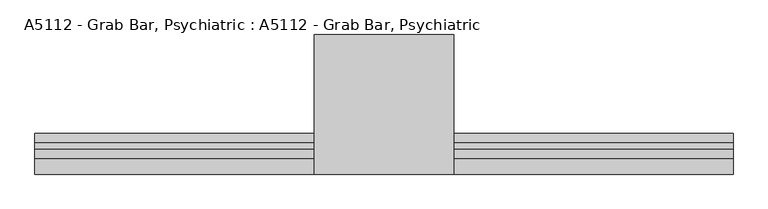
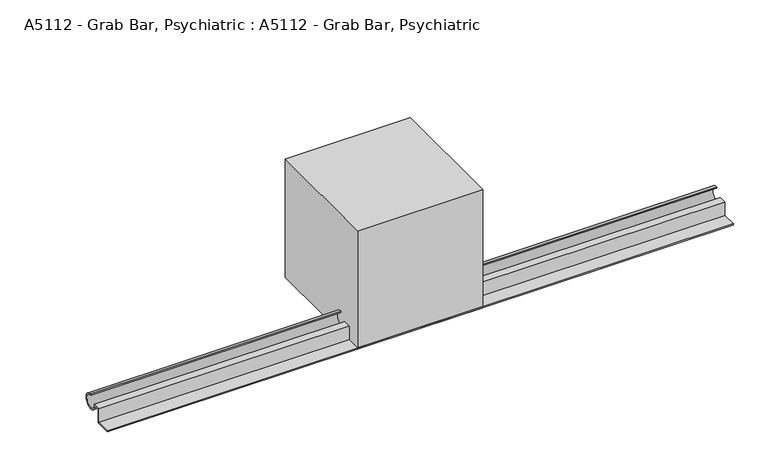
"""IFC4 building model written with IfcOpenShell, lengths in millimetres: proxy geometry, A5112 - Grab Bar, Psychiatric : A5112 - Grab Bar, Psychiatric."""

import ifcopenshell
import ifcopenshell.guid

model = None  # the IFC model being written
_history = None  # IfcOwnerHistory: only IFC2X3 demands one
_inside = {}  # id of a spatial element -> (the spatial element, [elements in it])
_under = {}  # id of a project, library or spatial element -> (it, [spatial elements below it])
_declared = {}  # id of a project -> (the project, [libraries it declares])
_typed = {}  # id of a type object -> (the type object, [elements of that type])
_made_of = {}  # id of a material, layer set ... -> (it, [elements and type objects made of it])


def new_model(schema):
    """Start an empty IFC model of exactly this schema.

    Asked for "IFC4X3", IfcOpenShell would pick the latest addendum, in which some entities
    have other attributes; the version numbers below select the first issue.
    IFC2X3 requires an IfcOwnerHistory on every rooted entity: one is made here for all.
    """
    global model, _history
    if schema == "IFC4X3":
        model = ifcopenshell.file(schema_version=(4, 3, 0, 0))
    else:
        model = ifcopenshell.file(schema=schema)
    _inside.clear()
    _under.clear()
    _declared.clear()
    _typed.clear()
    _made_of.clear()
    _history = None
    if model.schema == "IFC2X3":
        org = make("IfcOrganization", Name="unknown")
        user = make(
            "IfcPersonAndOrganization",
            ThePerson=make("IfcPerson", FamilyName="unknown"),
            TheOrganization=org,
        )
        app = make(
            "IfcApplication",
            ApplicationDeveloper=org,
            Version="unknown",
            ApplicationFullName="unknown",
            ApplicationIdentifier="unknown",
        )
        _history = make(
            "IfcOwnerHistory",
            OwningUser=user,
            OwningApplication=app,
            ChangeAction="ADDED",
            CreationDate=0,
        )
    return model


def make(cls, **values):
    """One entity of the class cls with the attributes given. An attribute that is None is left unset."""
    return model.create_entity(
        cls, **{name: value for name, value in values.items() if value is not None}
    )


def rooted(cls, **values):
    """An entity with a GlobalId (a new one), such as an element, a storey or a relation."""
    return make(cls, GlobalId=ifcopenshell.guid.new(), OwnerHistory=_history, **values)


def si_unit(unit_type, name, prefix=None):
    """IfcSIUnit, for example si_unit("LENGTHUNIT", "METRE", prefix="MILLI")."""
    return make("IfcSIUnit", UnitType=unit_type, Prefix=prefix, Name=name)


def assignment(units):
    """IfcUnitAssignment: the units of a project."""
    return None if units is None else make("IfcUnitAssignment", Units=units)


def point(xyz):
    """IfcCartesianPoint."""
    return None if xyz is None else make("IfcCartesianPoint", Coordinates=xyz)


def direction(xyz):
    """IfcDirection."""
    return None if xyz is None else make("IfcDirection", DirectionRatios=xyz)


def frame(location, z_axis=None, x_axis=None):
    """IfcAxis2Placement3D, a coordinate frame: its origin and axes. An axis left out is left unset."""
    return make(
        "IfcAxis2Placement3D",
        Location=point(location),
        Axis=direction(z_axis),
        RefDirection=direction(x_axis),
    )


def frame_2d(location, x_axis=None):
    """IfcAxis2Placement2D, a coordinate frame in the plane: its origin and x axis."""
    return make(
        "IfcAxis2Placement2D", Location=point(location), RefDirection=direction(x_axis)
    )


def origin():
    """The frame at (0, 0, 0) with its axes left unset."""
    return frame((0.0, 0.0, 0.0))


def origin_with_axes():
    """The frame at (0, 0, 0) with the z axis (0, 0, 1) and the x axis (1, 0, 0) written out."""
    return frame((0.0, 0.0, 0.0), z_axis=(0.0, 0.0, 1.0), x_axis=(1.0, 0.0, 0.0))


def place(relative_to, where):
    """IfcLocalPlacement: puts the frame where relative to a parent placement (None: the world)."""
    return make(
        "IfcLocalPlacement", PlacementRelTo=relative_to, RelativePlacement=where
    )


def context(
    kind, dimensions, precision=None, world=None, true_north=None, identifier=None
):
    """IfcGeometricRepresentationContext, for example the 3D "Model" context."""
    return make(
        "IfcGeometricRepresentationContext",
        ContextIdentifier=identifier,
        ContextType=kind,
        CoordinateSpaceDimension=dimensions,
        Precision=precision,
        WorldCoordinateSystem=world,
        TrueNorth=true_north,
    )


def project(units=None, contexts=None):
    """IfcProject with its units and contexts."""
    return rooted(
        "IfcProject",
        Name="project",
        RepresentationContexts=contexts,
        UnitsInContext=assignment(units),
    )


def spatial(cls, under=None, at=None, **own):
    """A site, building, storey or space (cls), placed at a placement, below another one or the project."""
    s = rooted(cls, ObjectPlacement=at, **own)
    if under is not None:
        _under.setdefault(under.id(), (under, []))[1].append(s)
    return s


def polyline(points):
    """IfcPolyline through the points."""
    return make("IfcPolyline", Points=[point(p) for p in points])


def circle_curve(where, radius):
    """IfcCircle in the frame where."""
    return make("IfcCircle", Position=where, Radius=radius)


def trimmed(basis, trim1, trim2, sense, master):
    """IfcTrimmedCurve: the piece of a basis curve between two trims."""
    return make(
        "IfcTrimmedCurve",
        BasisCurve=basis,
        Trim1=trim1,
        Trim2=trim2,
        SenseAgreement=sense,
        MasterRepresentation=master,
    )


def segment(curve, same_sense, transition):
    """IfcCompositeCurveSegment."""
    return make(
        "IfcCompositeCurveSegment",
        Transition=transition,
        SameSense=same_sense,
        ParentCurve=curve,
    )


def composite_curve(segments, self_intersect=None):
    """IfcCompositeCurve: segments joined end to end."""
    return make("IfcCompositeCurve", Segments=segments, SelfIntersect=self_intersect)


def outline(outer, holes=None, kind="AREA"):
    """IfcArbitraryClosedProfileDef: a profile drawn as a closed curve; with holes, ...WithVoids."""
    if holes is None:
        return make("IfcArbitraryClosedProfileDef", ProfileType=kind, OuterCurve=outer)
    return make(
        "IfcArbitraryProfileDefWithVoids",
        ProfileType=kind,
        OuterCurve=outer,
        InnerCurves=holes,
    )


def extrude(swept, where, along, depth):
    """IfcExtrudedAreaSolid: the profile swept, set in the frame where, extruded along a direction by depth."""
    return make(
        "IfcExtrudedAreaSolid",
        SweptArea=swept,
        Position=where,
        ExtrudedDirection=direction(along),
        Depth=depth,
    )


def shape(context_of_items, identifier, shape_type, items):
    """IfcShapeRepresentation: the items that make up one representation, for example the "Body"."""
    return make(
        "IfcShapeRepresentation",
        ContextOfItems=context_of_items,
        RepresentationIdentifier=identifier,
        RepresentationType=shape_type,
        Items=items,
    )


def source(mapping_origin, context_of_items, identifier, shape_type, items):
    """IfcRepresentationMap: a shape defined once, which mapped items show again and again."""
    return make(
        "IfcRepresentationMap",
        MappingOrigin=mapping_origin,
        MappedRepresentation=shape(context_of_items, identifier, shape_type, items),
    )


def transform(
    local_origin,
    x_axis=None,
    y_axis=None,
    z_axis=None,
    scale=None,
    scale2=None,
    scale3=None,
    uniform=True,
):
    """IfcCartesianTransformationOperator3D, or its non-uniform kind. x_axis, y_axis, z_axis: its Axis1, 2, 3."""
    if uniform:
        return make(
            "IfcCartesianTransformationOperator3D",
            Axis1=direction(x_axis),
            Axis2=direction(y_axis),
            LocalOrigin=point(local_origin),
            Scale=scale,
            Axis3=direction(z_axis),
        )
    return make(
        "IfcCartesianTransformationOperator3DnonUniform",
        Axis1=direction(x_axis),
        Axis2=direction(y_axis),
        LocalOrigin=point(local_origin),
        Scale=scale,
        Axis3=direction(z_axis),
        Scale2=scale2,
        Scale3=scale3,
    )


def mapped(mapping_source, mapping_target):
    """IfcMappedItem: shows the shape of a source again, moved by a transform."""
    return make(
        "IfcMappedItem", MappingSource=mapping_source, MappingTarget=mapping_target
    )


def made_of(thing, what):
    """Note that an element or type object is made of a material, layer set ...; save() writes the relation."""
    if what is not None:
        _made_of.setdefault(what.id(), (what, []))[1].append(thing)
    return thing


def element(
    cls,
    number,
    at=None,
    inside=None,
    cuts=None,
    type_object=None,
    material=None,
    context=None,
    identifier="Body",
    shape_type=None,
    held_by="IfcProductDefinitionShape",
    body=None,
    shapes=None,
    **own,
):
    """One element of the class cls, such as IfcWall. Its Tag is "e" and its number.

    at: its placement. inside: the storey or other place that contains it. cuts: it is an
    opening in that element (IfcRelVoidsElement). A single representation is given by context,
    identifier, shape_type and body (its items); several are given by shapes. held_by: the class
    of the entity that holds the representations. save() writes the other relations.
    """
    e = rooted(cls, Tag="e%d" % number, ObjectPlacement=at, **own)
    if body is not None:
        shapes = [shape(context, identifier, shape_type, body)]
    if shapes is not None:
        e.Representation = make(held_by, Representations=shapes)
    if inside is not None:
        _inside.setdefault(inside.id(), (inside, []))[1].append(e)
    if cuts is not None:
        rooted(
            "IfcRelVoidsElement", RelatingBuildingElement=cuts, RelatedOpeningElement=e
        )
    if type_object is not None:
        _typed.setdefault(type_object.id(), (type_object, []))[1].append(e)
    return made_of(e, material)


def aggregate(whole, parts):
    """IfcRelAggregates: a whole, such as a stair, and the parts it consists of."""
    return rooted("IfcRelAggregates", RelatingObject=whole, RelatedObjects=parts)


def save(model, path):
    """Write the relations noted so far, then the file.

    IfcRelAggregates (storeys below a building ...), IfcRelContainedInSpatialStructure (elements
    in a storey), IfcRelDefinesByType, IfcRelAssociatesMaterial and IfcRelDeclares: one each for
    every whole, place, type object, material and project.
    """
    for whole, parts in _under.values():
        aggregate(whole, parts)
    for where, things in _inside.values():
        rooted(
            "IfcRelContainedInSpatialStructure",
            RelatedElements=things,
            RelatingStructure=where,
        )
    for kind, things in _typed.values():
        rooted("IfcRelDefinesByType", RelatedObjects=things, RelatingType=kind)
    for what, things in _made_of.values():
        rooted("IfcRelAssociatesMaterial", RelatedObjects=things, RelatingMaterial=what)
    for by, libraries in _declared.values():
        rooted("IfcRelDeclares", RelatingContext=by, RelatedDefinitions=libraries)
    model.write(path)


def a5112_grab_bar_psychiatric_a5112_grab_bar_psychiatric_dcd99951(model_context):
    return source(origin(), model_context, "Body", "SweptSolid", [
        extrude(outline(composite_curve([segment(polyline([(38.1, 0.0), (0.0, 0.0), (0.0, 3.175), (34.925, 3.175), (34.925, 38.1), (54.0545744, 38.1)]), True, "CONTINUOUS"), segment(trimmed(circle_curve(frame_2d((69.85, 36.5125)), 15.875), [point((54.0545744, 38.1))], [point((69.85, 52.3875))], True, "CARTESIAN"), True, "CONTINUOUS"), segment(polyline([(69.85, 52.3875), (69.85, 55.5625)]), True, "CONTINUOUS"), segment(trimmed(circle_curve(frame_2d((69.85, 36.5125)), 19.05), [point((69.85, 55.5625))], [point((50.8662611, 34.925))], False, "CARTESIAN"), True, "CONTINUOUS"), segment(polyline([(50.8662611, 34.925), (38.1, 34.925), (38.1, 0.0)]), True, "CONTINUOUS")], self_intersect=False)), frame((-762.0, 0.0, 0.0), z_axis=(1.0, 0.0, 0.0), x_axis=(0.0, 1.0, 0.0)), (0.0, 0.0, 1.0), 1524.0),
        extrude(outline(polyline([(152.4, 304.8), (152.4, 0.0), (-152.4, 0.0), (-152.4, 304.8), (152.4, 304.8)])), origin_with_axes(), (0.0, 0.0, 1.0), 304.8),
    ])


if __name__ == "__main__":
    model = new_model("IFC4")
    model_context = context("Model", 3, world=origin())
    ifc_project = project(units=[si_unit("LENGTHUNIT", "METRE", prefix="MILLI")], contexts=[model_context])
    site = spatial("IfcSite", under=ifc_project)
    building = spatial("IfcBuilding", under=site)
    placement = place(None, origin())
    a5112_grab_bar_psychiatric_a5112_grab_bar_psychiatric_shape = a5112_grab_bar_psychiatric_a5112_grab_bar_psychiatric_dcd99951(model_context)
    element("IfcBuildingElementProxy", 1, Name="A5112 - Grab Bar, Psychiatric : A5112 - Grab Bar, Psychiatric", ObjectType="A5112 - Grab Bar, Psychiatric : A5112 - Grab Bar, Psychiatric", at=placement, inside=building, context=model_context, shape_type="MappedRepresentation", body=[
        mapped(a5112_grab_bar_psychiatric_a5112_grab_bar_psychiatric_shape, transform((0.0, 0.0, 0.0), x_axis=(1.0, 0.0, 0.0), y_axis=(0.0, 1.0, 0.0), z_axis=(0.0, 0.0, 1.0))),
    ])
    save(model, "model.ifc")

# Revit data of these elements
# Type "A5112 - Grab Bar, Psychiatric : A5112 - Grab Bar, Psychiatric"
#   Watts2 = "0"
#   Watts1 = "0"
#   Unit_Issue = "EA"
#   UTIL_6_Misc = "-"
#   UTIL_5_NonMedGas = "-"
#   UTIL_4_MiscGas = "-"
#   UTIL_3_MedGas = "-"
#   UTIL_2_Elec = "-"
#   UTIL_1_WaterDrain = "-"
#   Nomenclature = "Grab Bar, Psychiatric"
#   NSN = ""
#   Location [instance default] = ""
#   JSN = "A5112"
#   Fund_Source_VA = "-"
#   Fund_Source_Navy = "-"
#   Fund_Source_Army = "-"
#   Fund_Source_AF = "-"
#   ELEC_Volts2 = "0"
#   ELEC_Volts1 = "0"
#   ELEC_Phase2 = "0"
#   ELEC_Phase1 = "0"
#   ELEC_HertzSwitch = "0"
#   ELEC_HertzDependent = "0"
#   ELEC_Hertz = "0"
#   ELEC_Amps2 = "0"
#   ELEC_Amps1 = "0"
#   DetailDescription = ""
#   CAT_VA = "A"
#   CAT_Navy = "A"
#   CAT_IHS = "-"
#   CAT_Army = "A"
#   CAT_AF = "A"
#   BTUperhour = "0"
#   Weight_IP = 0
#   DIM_Width_IP = 1' - 0"
#   DIM_Height_IP = 1' - 0"
#   DIM_Depth_IP = 1' - 0"
#   CustomLength [instance default] = 2' - 0"
#   Default Elevation = 0
# Element 1 (IfcBuildingElementProxy, "A5112 - Grab Bar, Psychiatric : A5112 - Grab Bar, Psychiatric")
#   Location = "TLTP2"
#   CustomLength = 5' - 0"
#   Materials on its faces: "EquipSpace"
# Materials
#   "EquipSpace": class "Unassigned", colour RGB 221 217 195, transparency 0.5
